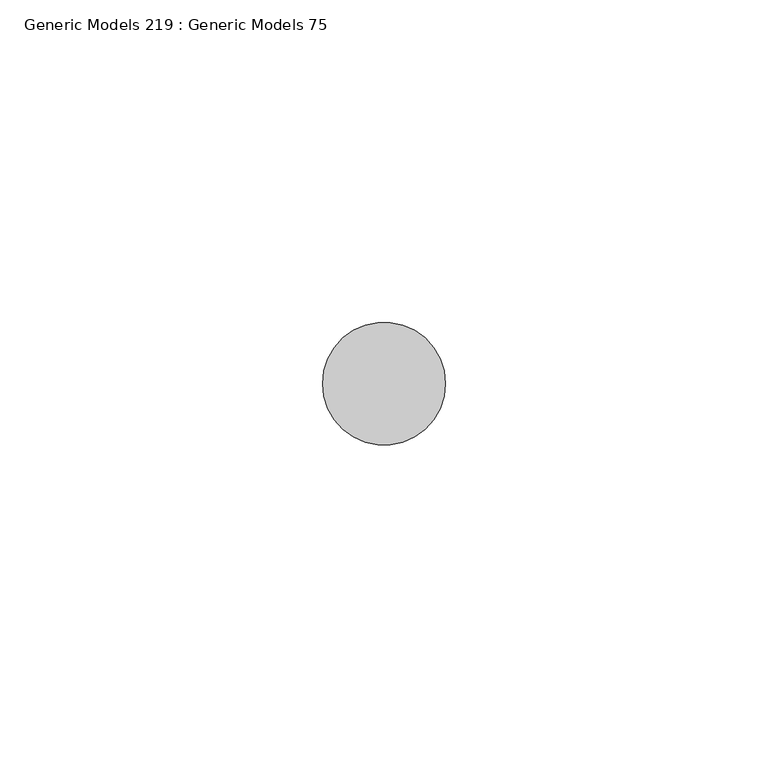
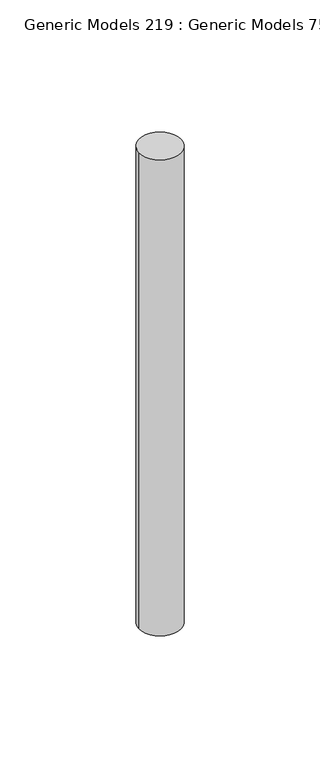
"""IFC4 building model written with IfcOpenShell, lengths in millimetres: proxy geometry, Generic Models 219 : Generic Models 75."""

from ifc_helpers import new_model, si_unit, point, frame, frame_2d, origin, place, context, project, spatial, circle_curve, trimmed, segment, composite_curve, outline, extrude, source, transform, mapped, element, save


def generic_models_219_generic_models_75_87fe1e97(model_context):
    return source(origin(), model_context, "Body", "SweptSolid", [
        extrude(outline(composite_curve([segment(trimmed(circle_curve(frame_2d((31988.1215778, 30896.6257369)), 9.525), [point((31978.5965778, 30896.6257369))], [point((31997.6465778, 30896.6257369))], False, "CARTESIAN"), True, "CONTINUOUS"), segment(trimmed(circle_curve(frame_2d((31988.1215778, 30896.6257369)), 9.525), [point((31997.6465778, 30896.6257369))], [point((31978.5965778, 30896.6257369))], False, "CARTESIAN"), True, "CONTINUOUS")], self_intersect=False)), frame((0.0, 0.0, 266211.05), z_axis=(0.0, 0.0, 1.0), x_axis=(1.0, 0.0, 0.0)), (0.0, 0.0, 1.0), 228.6),
    ])


if __name__ == "__main__":
    model = new_model("IFC4")
    model_context = context("Model", 3, world=origin())
    ifc_project = project(units=[si_unit("LENGTHUNIT", "METRE", prefix="MILLI")], contexts=[model_context])
    site = spatial("IfcSite", under=ifc_project)
    building = spatial("IfcBuilding", under=site)
    placement = place(None, origin())
    generic_models_219_generic_models_75_shape = generic_models_219_generic_models_75_87fe1e97(model_context)
    element("IfcBuildingElementProxy", 1, Name="Generic Models 219 : Generic Models 75", ObjectType="Generic Models 219 : Generic Models 75", at=placement, inside=building, context=model_context, shape_type="MappedRepresentation", body=[
        mapped(generic_models_219_generic_models_75_shape, transform((0.0, 0.0, 0.0), x_axis=(1.0, 0.0, 0.0), y_axis=(0.0, 1.0, 0.0), z_axis=(0.0, 0.0, 1.0))),
    ])
    save(model, "model.ifc")

# Revit data of these elements
# Element 1 (IfcBuildingElementProxy, "Generic Models 219 : Generic Models 75")
#   Materials on its faces: "5/8\" DIA. EPOXY ANCHOR BOLTS"
# Materials
#   "5/8\" DIA. EPOXY ANCHOR BOLTS": class "Metal", colour RGB 199 199 199, transparency 0, Description = "Carbon steel", Cost = 0
